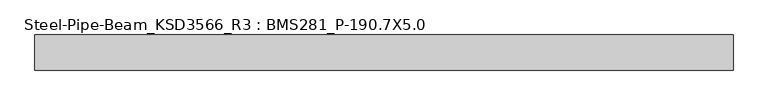
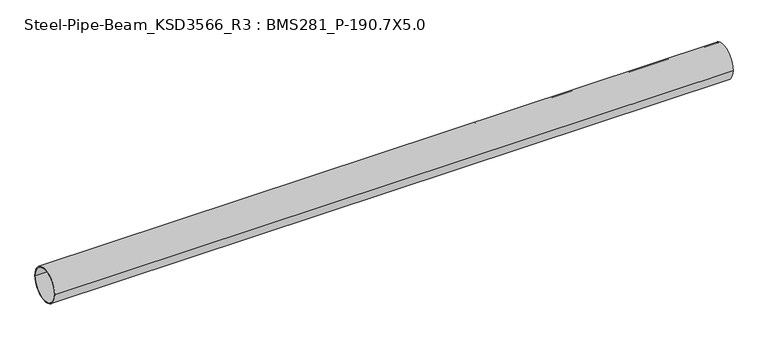
"""IFC4 building model written with IfcOpenShell, lengths in millimetres: member geometry, Steel-Pipe-Beam_KSD3566_R3 : BMS281_P-190.7X5.0."""

from ifc_helpers import new_model, si_unit, point, frame, origin, origin_2d, place, context, project, spatial, circle_curve, trimmed, segment, composite_curve, outline, extrude, source, transform, mapped, element, save


def steel_pipe_beam_ksd3566_r3_bms281_p_190_7x5_0_dda89568(model_context):
    return source(origin(), model_context, "Body", "SweptSolid", [
        extrude(outline(composite_curve([segment(trimmed(circle_curve(origin_2d(), 95.35), [point((-95.35, 0.0))], [point((95.35, 0.0))], False, "CARTESIAN"), True, "CONTINUOUS"), segment(trimmed(circle_curve(origin_2d(), 95.35), [point((95.35, 0.0))], [point((-95.35, 0.0))], False, "CARTESIAN"), True, "CONTINUOUS")], self_intersect=False), holes=[composite_curve([segment(trimmed(circle_curve(origin_2d(), 90.35), [point((90.35, 0.0))], [point((-90.35, 0.0))], True, "CARTESIAN"), True, "CONTINUOUS"), segment(trimmed(circle_curve(origin_2d(), 90.35), [point((-90.35, 0.0))], [point((90.35, 0.0))], True, "CARTESIAN"), True, "CONTINUOUS")], self_intersect=False)]), frame((-1901.3650173, 0.0, 0.0), z_axis=(1.0, 0.0, 0.0), x_axis=(0.0, 1.0, 0.0)), (0.0, 0.0, 1.0), 3789.2455083),
    ])


if __name__ == "__main__":
    model = new_model("IFC4")
    model_context = context("Model", 3, world=origin())
    ifc_project = project(units=[si_unit("LENGTHUNIT", "METRE", prefix="MILLI")], contexts=[model_context])
    site = spatial("IfcSite", under=ifc_project)
    building = spatial("IfcBuilding", under=site)
    placement = place(None, origin())
    steel_pipe_beam_ksd3566_r3_bms281_p_190_7x5_0_shape = steel_pipe_beam_ksd3566_r3_bms281_p_190_7x5_0_dda89568(model_context)
    element("IfcMember", 1, ObjectType="Steel-Pipe-Beam_KSD3566_R3 : BMS281_P-190.7X5.0", at=placement, inside=building, context=model_context, shape_type="MappedRepresentation", body=[
        mapped(steel_pipe_beam_ksd3566_r3_bms281_p_190_7x5_0_shape, transform((0.0, 0.0, 0.0), x_axis=(1.0, 0.0, 0.0), y_axis=(0.0, 1.0, 0.0), z_axis=(0.0, 0.0, 1.0))),
    ])
    save(model, "model.ifc")

# Revit data of these elements
# Type "Steel-Pipe-Beam_KSD3566_R3 : BMS281_P-190.7X5.0"
#   Keynote = "P-190.7X5.0"
#   SteelWeight = "Light"
#   t = 0.0050 m
#   Surface Area = 0.599102 m²/m
#   Section Area = 29.1697 cm²
#   Mass per Unit Length = 22.8982 kg/m
#   Length [instance default] = 1.5000 m
#   D = 0.1907 m
#   hec_material4 [instance default] = none
#   hec_material3 [instance default] = none
#   hec_material2 [instance default] = none
#   hec_material1 [instance default] = none
#   Structural Material [instance default] = Steel, 45-345
#   Assembly Code = ""
# Element 1 (IfcMember, "Steel-Pipe-Beam_KSD3566_R3 : BMS281_P-190.7X5.0")
#   Structural Material = none
# Materials
#   "Steel, 45-345": class "Metal", colour RGB 189 187 185, transparency 0, Description = "Steel 345 MPa", Cost = 0
